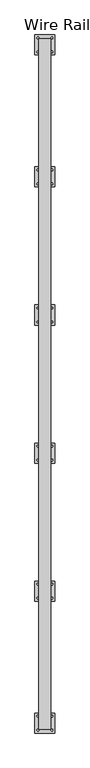
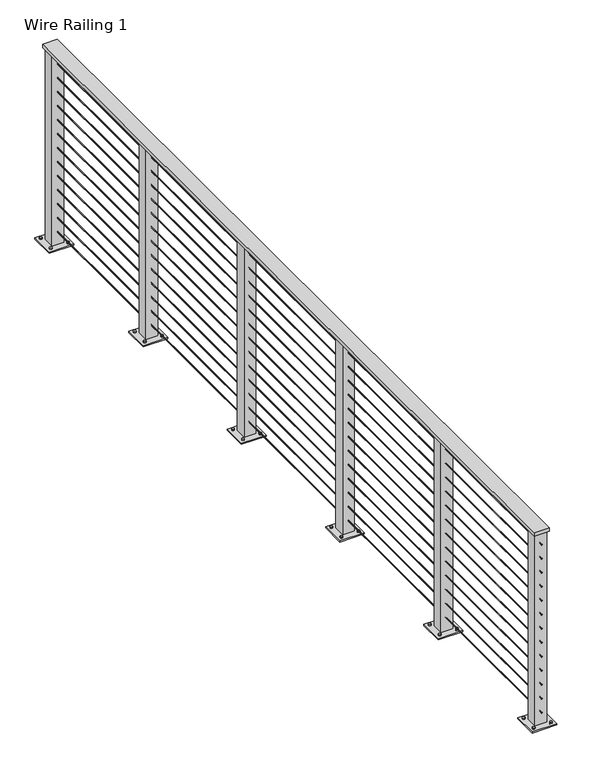
"""IFC4 building model written with IfcOpenShell, lengths in millimetres: railing geometry, Wire Railing 1."""

from ifc_helpers import new_model, si_unit, point, frame, frame_2d, origin, place, context, project, spatial, polyline, circle_curve, trimmed, segment, composite_curve, outline, extrude, source, transform, mapped, element, save


def wire_railing_1_9a376ef2(model_context):
    return source(origin(), model_context, "Body", "SweptSolid", [
        extrude(outline(polyline([(33186.6840778, 35259.9668167), (33262.8840778, 35259.9668167), (33262.8840778, 30878.4668167), (33186.6840778, 30878.4668167), (33186.6840778, 35259.9668167)])), frame((0.0, 0.0, 270300.45), z_axis=(0.0, 0.0, 1.0), x_axis=(1.0, 0.0, 0.0)), (0.0, 0.0, 1.0), 19.05),
        extrude(outline(composite_curve([segment(trimmed(circle_curve(frame_2d((270240.91875, 33224.7840778)), 2.38125), [point((270240.91875, 33227.1653278))], [point((270240.91875, 33222.4028278))], False, "CARTESIAN"), True, "CONTINUOUS"), segment(trimmed(circle_curve(frame_2d((270240.91875, 33224.7840778)), 2.38125), [point((270240.91875, 33222.4028278))], [point((270240.91875, 33227.1653278))], False, "CARTESIAN"), True, "CONTINUOUS")], self_intersect=False)), frame((0.0, 30878.4668167, 0.0), z_axis=(0.0, 1.0, 0.0), x_axis=(0.0, 0.0, 1.0)), (0.0, 0.0, 1.0), 4381.5),
        extrude(outline(composite_curve([segment(trimmed(circle_curve(frame_2d((270164.71875, 33224.7840778)), 2.38125), [point((270164.71875, 33227.1653278))], [point((270164.71875, 33222.4028278))], False, "CARTESIAN"), True, "CONTINUOUS"), segment(trimmed(circle_curve(frame_2d((270164.71875, 33224.7840778)), 2.38125), [point((270164.71875, 33222.4028278))], [point((270164.71875, 33227.1653278))], False, "CARTESIAN"), True, "CONTINUOUS")], self_intersect=False)), frame((0.0, 30878.4668167, 0.0), z_axis=(0.0, 1.0, 0.0), x_axis=(0.0, 0.0, 1.0)), (0.0, 0.0, 1.0), 4381.5),
        extrude(outline(composite_curve([segment(trimmed(circle_curve(frame_2d((270088.51875, 33224.7840778)), 2.38125), [point((270088.51875, 33227.1653278))], [point((270088.51875, 33222.4028278))], False, "CARTESIAN"), True, "CONTINUOUS"), segment(trimmed(circle_curve(frame_2d((270088.51875, 33224.7840778)), 2.38125), [point((270088.51875, 33222.4028278))], [point((270088.51875, 33227.1653278))], False, "CARTESIAN"), True, "CONTINUOUS")], self_intersect=False)), frame((0.0, 30878.4668167, 0.0), z_axis=(0.0, 1.0, 0.0), x_axis=(0.0, 0.0, 1.0)), (0.0, 0.0, 1.0), 4381.5),
        extrude(outline(composite_curve([segment(trimmed(circle_curve(frame_2d((270012.31875, 33224.7840778)), 2.38125), [point((270012.31875, 33227.1653278))], [point((270012.31875, 33222.4028278))], False, "CARTESIAN"), True, "CONTINUOUS"), segment(trimmed(circle_curve(frame_2d((270012.31875, 33224.7840778)), 2.38125), [point((270012.31875, 33222.4028278))], [point((270012.31875, 33227.1653278))], False, "CARTESIAN"), True, "CONTINUOUS")], self_intersect=False)), frame((0.0, 30878.4668167, 0.0), z_axis=(0.0, 1.0, 0.0), x_axis=(0.0, 0.0, 1.0)), (0.0, 0.0, 1.0), 4381.5),
        extrude(outline(composite_curve([segment(trimmed(circle_curve(frame_2d((269936.11875, 33224.7840778)), 2.38125), [point((269936.11875, 33227.1653278))], [point((269936.11875, 33222.4028278))], False, "CARTESIAN"), True, "CONTINUOUS"), segment(trimmed(circle_curve(frame_2d((269936.11875, 33224.7840778)), 2.38125), [point((269936.11875, 33222.4028278))], [point((269936.11875, 33227.1653278))], False, "CARTESIAN"), True, "CONTINUOUS")], self_intersect=False)), frame((0.0, 30878.4668167, 0.0), z_axis=(0.0, 1.0, 0.0), x_axis=(0.0, 0.0, 1.0)), (0.0, 0.0, 1.0), 4381.5),
        extrude(outline(composite_curve([segment(trimmed(circle_curve(frame_2d((269859.91875, 33224.7840778)), 2.38125), [point((269859.91875, 33227.1653278))], [point((269859.91875, 33222.4028278))], False, "CARTESIAN"), True, "CONTINUOUS"), segment(trimmed(circle_curve(frame_2d((269859.91875, 33224.7840778)), 2.38125), [point((269859.91875, 33222.4028278))], [point((269859.91875, 33227.1653278))], False, "CARTESIAN"), True, "CONTINUOUS")], self_intersect=False)), frame((0.0, 30878.4668167, 0.0), z_axis=(0.0, 1.0, 0.0), x_axis=(0.0, 0.0, 1.0)), (0.0, 0.0, 1.0), 4381.5),
        extrude(outline(composite_curve([segment(trimmed(circle_curve(frame_2d((269783.71875, 33224.7840778)), 2.38125), [point((269783.71875, 33227.1653278))], [point((269783.71875, 33222.4028278))], False, "CARTESIAN"), True, "CONTINUOUS"), segment(trimmed(circle_curve(frame_2d((269783.71875, 33224.7840778)), 2.38125), [point((269783.71875, 33222.4028278))], [point((269783.71875, 33227.1653278))], False, "CARTESIAN"), True, "CONTINUOUS")], self_intersect=False)), frame((0.0, 30878.4668167, 0.0), z_axis=(0.0, 1.0, 0.0), x_axis=(0.0, 0.0, 1.0)), (0.0, 0.0, 1.0), 4381.5),
        extrude(outline(composite_curve([segment(trimmed(circle_curve(frame_2d((269707.51875, 33224.7840778)), 2.38125), [point((269707.51875, 33227.1653278))], [point((269707.51875, 33222.4028278))], False, "CARTESIAN"), True, "CONTINUOUS"), segment(trimmed(circle_curve(frame_2d((269707.51875, 33224.7840778)), 2.38125), [point((269707.51875, 33222.4028278))], [point((269707.51875, 33227.1653278))], False, "CARTESIAN"), True, "CONTINUOUS")], self_intersect=False)), frame((0.0, 30878.4668167, 0.0), z_axis=(0.0, 1.0, 0.0), x_axis=(0.0, 0.0, 1.0)), (0.0, 0.0, 1.0), 4381.5),
        extrude(outline(composite_curve([segment(trimmed(circle_curve(frame_2d((269631.31875, 33224.7840778)), 2.38125), [point((269631.31875, 33227.1653278))], [point((269631.31875, 33222.4028278))], False, "CARTESIAN"), True, "CONTINUOUS"), segment(trimmed(circle_curve(frame_2d((269631.31875, 33224.7840778)), 2.38125), [point((269631.31875, 33222.4028278))], [point((269631.31875, 33227.1653278))], False, "CARTESIAN"), True, "CONTINUOUS")], self_intersect=False)), frame((0.0, 30878.4668167, 0.0), z_axis=(0.0, 1.0, 0.0), x_axis=(0.0, 0.0, 1.0)), (0.0, 0.0, 1.0), 4381.5),
        extrude(outline(composite_curve([segment(trimmed(circle_curve(frame_2d((269555.11875, 33224.7840778)), 2.38125), [point((269555.11875, 33227.1653278))], [point((269555.11875, 33222.4028278))], False, "CARTESIAN"), True, "CONTINUOUS"), segment(trimmed(circle_curve(frame_2d((269555.11875, 33224.7840778)), 2.38125), [point((269555.11875, 33222.4028278))], [point((269555.11875, 33227.1653278))], False, "CARTESIAN"), True, "CONTINUOUS")], self_intersect=False)), frame((0.0, 30878.4668167, 0.0), z_axis=(0.0, 1.0, 0.0), x_axis=(0.0, 0.0, 1.0)), (0.0, 0.0, 1.0), 4381.5),
        extrude(outline(composite_curve([segment(trimmed(circle_curve(frame_2d((269478.91875, 33224.7840778)), 2.38125), [point((269478.91875, 33227.1653278))], [point((269478.91875, 33222.4028278))], False, "CARTESIAN"), True, "CONTINUOUS"), segment(trimmed(circle_curve(frame_2d((269478.91875, 33224.7840778)), 2.38125), [point((269478.91875, 33222.4028278))], [point((269478.91875, 33227.1653278))], False, "CARTESIAN"), True, "CONTINUOUS")], self_intersect=False)), frame((0.0, 30878.4668167, 0.0), z_axis=(0.0, 1.0, 0.0), x_axis=(0.0, 0.0, 1.0)), (0.0, 0.0, 1.0), 4381.5),
        extrude(outline(composite_curve([segment(trimmed(circle_curve(frame_2d((269402.71875, 33224.7840778)), 2.38125), [point((269402.71875, 33227.1653278))], [point((269402.71875, 33222.4028278))], False, "CARTESIAN"), True, "CONTINUOUS"), segment(trimmed(circle_curve(frame_2d((269402.71875, 33224.7840778)), 2.38125), [point((269402.71875, 33222.4028278))], [point((269402.71875, 33227.1653278))], False, "CARTESIAN"), True, "CONTINUOUS")], self_intersect=False)), frame((0.0, 30878.4668167, 0.0), z_axis=(0.0, 1.0, 0.0), x_axis=(0.0, 0.0, 1.0)), (0.0, 0.0, 1.0), 4381.5),
        extrude(outline(composite_curve([segment(trimmed(circle_curve(frame_2d((269326.51875, 33224.7840778)), 2.38125), [point((269326.51875, 33227.1653278))], [point((269326.51875, 33222.4028278))], False, "CARTESIAN"), True, "CONTINUOUS"), segment(trimmed(circle_curve(frame_2d((269326.51875, 33224.7840778)), 2.38125), [point((269326.51875, 33222.4028278))], [point((269326.51875, 33227.1653278))], False, "CARTESIAN"), True, "CONTINUOUS")], self_intersect=False)), frame((0.0, 30878.4668167, 0.0), z_axis=(0.0, 1.0, 0.0), x_axis=(0.0, 0.0, 1.0)), (0.0, 0.0, 1.0), 4381.5),
        extrude(outline(composite_curve([segment(trimmed(circle_curve(frame_2d((33180.3340778, 31799.2168167)), 6.35), [point((33173.9840778, 31799.2168167))], [point((33186.6840778, 31799.2168167))], False, "CARTESIAN"), True, "CONTINUOUS"), segment(trimmed(circle_curve(frame_2d((33180.3340778, 31799.2168167)), 6.35), [point((33186.6840778, 31799.2168167))], [point((33173.9840778, 31799.2168167))], False, "CARTESIAN"), True, "CONTINUOUS")], self_intersect=False)), frame((0.0, 0.0, 269252.7), z_axis=(0.0, 0.0, 1.0), x_axis=(1.0, 0.0, 0.0)), (0.0, 0.0, 1.0), 12.7),
        extrude(outline(composite_curve([segment(trimmed(circle_curve(frame_2d((33269.2340778, 31799.2168167)), 6.35), [point((33262.8840778, 31799.2168167))], [point((33275.5840778, 31799.2168167))], False, "CARTESIAN"), True, "CONTINUOUS"), segment(trimmed(circle_curve(frame_2d((33269.2340778, 31799.2168167)), 6.35), [point((33275.5840778, 31799.2168167))], [point((33262.8840778, 31799.2168167))], False, "CARTESIAN"), True, "CONTINUOUS")], self_intersect=False)), frame((0.0, 0.0, 269252.7), z_axis=(0.0, 0.0, 1.0), x_axis=(1.0, 0.0, 0.0)), (0.0, 0.0, 1.0), 12.7),
        extrude(outline(composite_curve([segment(trimmed(circle_curve(frame_2d((33180.3340778, 31710.3168167)), 6.35), [point((33173.9840778, 31710.3168167))], [point((33186.6840778, 31710.3168167))], False, "CARTESIAN"), True, "CONTINUOUS"), segment(trimmed(circle_curve(frame_2d((33180.3340778, 31710.3168167)), 6.35), [point((33186.6840778, 31710.3168167))], [point((33173.9840778, 31710.3168167))], False, "CARTESIAN"), True, "CONTINUOUS")], self_intersect=False)), frame((0.0, 0.0, 269252.7), z_axis=(0.0, 0.0, 1.0), x_axis=(1.0, 0.0, 0.0)), (0.0, 0.0, 1.0), 12.7),
        extrude(outline(composite_curve([segment(trimmed(circle_curve(frame_2d((33269.2340778, 31710.3168167)), 6.35), [point((33262.8840778, 31710.3168167))], [point((33275.5840778, 31710.3168167))], False, "CARTESIAN"), True, "CONTINUOUS"), segment(trimmed(circle_curve(frame_2d((33269.2340778, 31710.3168167)), 6.35), [point((33275.5840778, 31710.3168167))], [point((33262.8840778, 31710.3168167))], False, "CARTESIAN"), True, "CONTINUOUS")], self_intersect=False)), frame((0.0, 0.0, 269252.7), z_axis=(0.0, 0.0, 1.0), x_axis=(1.0, 0.0, 0.0)), (0.0, 0.0, 1.0), 12.7),
        extrude(outline(polyline([(33288.2840778, 31818.2668167), (33288.2840778, 31691.2668167), (33161.2840778, 31691.2668167), (33161.2840778, 31818.2668167), (33288.2840778, 31818.2668167)])), frame((0.0, 0.0, 269252.7), z_axis=(0.0, 0.0, 1.0), x_axis=(1.0, 0.0, 0.0)), (0.0, 0.0, 1.0), 6.35),
        extrude(outline(polyline([(33254.9465778, 31784.9293167), (33254.9465778, 31724.6043167), (33194.6215778, 31724.6043167), (33194.6215778, 31784.9293167), (33254.9465778, 31784.9293167)]), holes=[polyline([(33248.5965778, 31778.5793167), (33200.9715778, 31778.5793167), (33200.9715778, 31730.9543167), (33248.5965778, 31730.9543167), (33248.5965778, 31778.5793167)])]), frame((0.0, 0.0, 269252.7), z_axis=(0.0, 0.0, 1.0), x_axis=(1.0, 0.0, 0.0)), (0.0, 0.0, 1.0), 1047.75),
        extrude(outline(composite_curve([segment(trimmed(circle_curve(frame_2d((33180.3340778, 32675.5168167)), 6.35), [point((33173.9840778, 32675.5168167))], [point((33186.6840778, 32675.5168167))], False, "CARTESIAN"), True, "CONTINUOUS"), segment(trimmed(circle_curve(frame_2d((33180.3340778, 32675.5168167)), 6.35), [point((33186.6840778, 32675.5168167))], [point((33173.9840778, 32675.5168167))], False, "CARTESIAN"), True, "CONTINUOUS")], self_intersect=False)), frame((0.0, 0.0, 269252.7), z_axis=(0.0, 0.0, 1.0), x_axis=(1.0, 0.0, 0.0)), (0.0, 0.0, 1.0), 12.7),
        extrude(outline(composite_curve([segment(trimmed(circle_curve(frame_2d((33269.2340778, 32675.5168167)), 6.35), [point((33262.8840778, 32675.5168167))], [point((33275.5840778, 32675.5168167))], False, "CARTESIAN"), True, "CONTINUOUS"), segment(trimmed(circle_curve(frame_2d((33269.2340778, 32675.5168167)), 6.35), [point((33275.5840778, 32675.5168167))], [point((33262.8840778, 32675.5168167))], False, "CARTESIAN"), True, "CONTINUOUS")], self_intersect=False)), frame((0.0, 0.0, 269252.7), z_axis=(0.0, 0.0, 1.0), x_axis=(1.0, 0.0, 0.0)), (0.0, 0.0, 1.0), 12.7),
        extrude(outline(composite_curve([segment(trimmed(circle_curve(frame_2d((33180.3340778, 32586.6168167)), 6.35), [point((33173.9840778, 32586.6168167))], [point((33186.6840778, 32586.6168167))], False, "CARTESIAN"), True, "CONTINUOUS"), segment(trimmed(circle_curve(frame_2d((33180.3340778, 32586.6168167)), 6.35), [point((33186.6840778, 32586.6168167))], [point((33173.9840778, 32586.6168167))], False, "CARTESIAN"), True, "CONTINUOUS")], self_intersect=False)), frame((0.0, 0.0, 269252.7), z_axis=(0.0, 0.0, 1.0), x_axis=(1.0, 0.0, 0.0)), (0.0, 0.0, 1.0), 12.7),
        extrude(outline(composite_curve([segment(trimmed(circle_curve(frame_2d((33269.2340778, 32586.6168167)), 6.35), [point((33262.8840778, 32586.6168167))], [point((33275.5840778, 32586.6168167))], False, "CARTESIAN"), True, "CONTINUOUS"), segment(trimmed(circle_curve(frame_2d((33269.2340778, 32586.6168167)), 6.35), [point((33275.5840778, 32586.6168167))], [point((33262.8840778, 32586.6168167))], False, "CARTESIAN"), True, "CONTINUOUS")], self_intersect=False)), frame((0.0, 0.0, 269252.7), z_axis=(0.0, 0.0, 1.0), x_axis=(1.0, 0.0, 0.0)), (0.0, 0.0, 1.0), 12.7),
        extrude(outline(polyline([(33288.2840778, 32694.5668167), (33288.2840778, 32567.5668167), (33161.2840778, 32567.5668167), (33161.2840778, 32694.5668167), (33288.2840778, 32694.5668167)])), frame((0.0, 0.0, 269252.7), z_axis=(0.0, 0.0, 1.0), x_axis=(1.0, 0.0, 0.0)), (0.0, 0.0, 1.0), 6.35),
        extrude(outline(polyline([(33254.9465778, 32661.2293167), (33254.9465778, 32600.9043167), (33194.6215778, 32600.9043167), (33194.6215778, 32661.2293167), (33254.9465778, 32661.2293167)]), holes=[polyline([(33248.5965778, 32654.8793167), (33200.9715778, 32654.8793167), (33200.9715778, 32607.2543167), (33248.5965778, 32607.2543167), (33248.5965778, 32654.8793167)])]), frame((0.0, 0.0, 269252.7), z_axis=(0.0, 0.0, 1.0), x_axis=(1.0, 0.0, 0.0)), (0.0, 0.0, 1.0), 1047.75),
        extrude(outline(composite_curve([segment(trimmed(circle_curve(frame_2d((33180.3340778, 33551.8168167)), 6.35), [point((33173.9840778, 33551.8168167))], [point((33186.6840778, 33551.8168167))], False, "CARTESIAN"), True, "CONTINUOUS"), segment(trimmed(circle_curve(frame_2d((33180.3340778, 33551.8168167)), 6.35), [point((33186.6840778, 33551.8168167))], [point((33173.9840778, 33551.8168167))], False, "CARTESIAN"), True, "CONTINUOUS")], self_intersect=False)), frame((0.0, 0.0, 269252.7), z_axis=(0.0, 0.0, 1.0), x_axis=(1.0, 0.0, 0.0)), (0.0, 0.0, 1.0), 12.7),
        extrude(outline(composite_curve([segment(trimmed(circle_curve(frame_2d((33269.2340778, 33551.8168167)), 6.35), [point((33262.8840778, 33551.8168167))], [point((33275.5840778, 33551.8168167))], False, "CARTESIAN"), True, "CONTINUOUS"), segment(trimmed(circle_curve(frame_2d((33269.2340778, 33551.8168167)), 6.35), [point((33275.5840778, 33551.8168167))], [point((33262.8840778, 33551.8168167))], False, "CARTESIAN"), True, "CONTINUOUS")], self_intersect=False)), frame((0.0, 0.0, 269252.7), z_axis=(0.0, 0.0, 1.0), x_axis=(1.0, 0.0, 0.0)), (0.0, 0.0, 1.0), 12.7),
        extrude(outline(composite_curve([segment(trimmed(circle_curve(frame_2d((33180.3340778, 33462.9168167)), 6.35), [point((33173.9840778, 33462.9168167))], [point((33186.6840778, 33462.9168167))], False, "CARTESIAN"), True, "CONTINUOUS"), segment(trimmed(circle_curve(frame_2d((33180.3340778, 33462.9168167)), 6.35), [point((33186.6840778, 33462.9168167))], [point((33173.9840778, 33462.9168167))], False, "CARTESIAN"), True, "CONTINUOUS")], self_intersect=False)), frame((0.0, 0.0, 269252.7), z_axis=(0.0, 0.0, 1.0), x_axis=(1.0, 0.0, 0.0)), (0.0, 0.0, 1.0), 12.7),
        extrude(outline(composite_curve([segment(trimmed(circle_curve(frame_2d((33269.2340778, 33462.9168167)), 6.35), [point((33262.8840778, 33462.9168167))], [point((33275.5840778, 33462.9168167))], False, "CARTESIAN"), True, "CONTINUOUS"), segment(trimmed(circle_curve(frame_2d((33269.2340778, 33462.9168167)), 6.35), [point((33275.5840778, 33462.9168167))], [point((33262.8840778, 33462.9168167))], False, "CARTESIAN"), True, "CONTINUOUS")], self_intersect=False)), frame((0.0, 0.0, 269252.7), z_axis=(0.0, 0.0, 1.0), x_axis=(1.0, 0.0, 0.0)), (0.0, 0.0, 1.0), 12.7),
        extrude(outline(polyline([(33288.2840778, 33570.8668167), (33288.2840778, 33443.8668167), (33161.2840778, 33443.8668167), (33161.2840778, 33570.8668167), (33288.2840778, 33570.8668167)])), frame((0.0, 0.0, 269252.7), z_axis=(0.0, 0.0, 1.0), x_axis=(1.0, 0.0, 0.0)), (0.0, 0.0, 1.0), 6.35),
        extrude(outline(polyline([(33254.9465778, 33537.5293167), (33254.9465778, 33477.2043167), (33194.6215778, 33477.2043167), (33194.6215778, 33537.5293167), (33254.9465778, 33537.5293167)]), holes=[polyline([(33248.5965778, 33531.1793167), (33200.9715778, 33531.1793167), (33200.9715778, 33483.5543167), (33248.5965778, 33483.5543167), (33248.5965778, 33531.1793167)])]), frame((0.0, 0.0, 269252.7), z_axis=(0.0, 0.0, 1.0), x_axis=(1.0, 0.0, 0.0)), (0.0, 0.0, 1.0), 1047.75),
        extrude(outline(composite_curve([segment(trimmed(circle_curve(frame_2d((33180.3340778, 34428.1168167)), 6.35), [point((33173.9840778, 34428.1168167))], [point((33186.6840778, 34428.1168167))], False, "CARTESIAN"), True, "CONTINUOUS"), segment(trimmed(circle_curve(frame_2d((33180.3340778, 34428.1168167)), 6.35), [point((33186.6840778, 34428.1168167))], [point((33173.9840778, 34428.1168167))], False, "CARTESIAN"), True, "CONTINUOUS")], self_intersect=False)), frame((0.0, 0.0, 269252.7), z_axis=(0.0, 0.0, 1.0), x_axis=(1.0, 0.0, 0.0)), (0.0, 0.0, 1.0), 12.7),
        extrude(outline(composite_curve([segment(trimmed(circle_curve(frame_2d((33269.2340778, 34428.1168167)), 6.35), [point((33262.8840778, 34428.1168167))], [point((33275.5840778, 34428.1168167))], False, "CARTESIAN"), True, "CONTINUOUS"), segment(trimmed(circle_curve(frame_2d((33269.2340778, 34428.1168167)), 6.35), [point((33275.5840778, 34428.1168167))], [point((33262.8840778, 34428.1168167))], False, "CARTESIAN"), True, "CONTINUOUS")], self_intersect=False)), frame((0.0, 0.0, 269252.7), z_axis=(0.0, 0.0, 1.0), x_axis=(1.0, 0.0, 0.0)), (0.0, 0.0, 1.0), 12.7),
        extrude(outline(composite_curve([segment(trimmed(circle_curve(frame_2d((33180.3340778, 34339.2168167)), 6.35), [point((33173.9840778, 34339.2168167))], [point((33186.6840778, 34339.2168167))], False, "CARTESIAN"), True, "CONTINUOUS"), segment(trimmed(circle_curve(frame_2d((33180.3340778, 34339.2168167)), 6.35), [point((33186.6840778, 34339.2168167))], [point((33173.9840778, 34339.2168167))], False, "CARTESIAN"), True, "CONTINUOUS")], self_intersect=False)), frame((0.0, 0.0, 269252.7), z_axis=(0.0, 0.0, 1.0), x_axis=(1.0, 0.0, 0.0)), (0.0, 0.0, 1.0), 12.7),
        extrude(outline(composite_curve([segment(trimmed(circle_curve(frame_2d((33269.2340778, 34339.2168167)), 6.35), [point((33262.8840778, 34339.2168167))], [point((33275.5840778, 34339.2168167))], False, "CARTESIAN"), True, "CONTINUOUS"), segment(trimmed(circle_curve(frame_2d((33269.2340778, 34339.2168167)), 6.35), [point((33275.5840778, 34339.2168167))], [point((33262.8840778, 34339.2168167))], False, "CARTESIAN"), True, "CONTINUOUS")], self_intersect=False)), frame((0.0, 0.0, 269252.7), z_axis=(0.0, 0.0, 1.0), x_axis=(1.0, 0.0, 0.0)), (0.0, 0.0, 1.0), 12.7),
        extrude(outline(polyline([(33288.2840778, 34447.1668167), (33288.2840778, 34320.1668167), (33161.2840778, 34320.1668167), (33161.2840778, 34447.1668167), (33288.2840778, 34447.1668167)])), frame((0.0, 0.0, 269252.7), z_axis=(0.0, 0.0, 1.0), x_axis=(1.0, 0.0, 0.0)), (0.0, 0.0, 1.0), 6.35),
        extrude(outline(polyline([(33254.9465778, 34413.8293167), (33254.9465778, 34353.5043167), (33194.6215778, 34353.5043167), (33194.6215778, 34413.8293167), (33254.9465778, 34413.8293167)]), holes=[polyline([(33248.5965778, 34407.4793167), (33200.9715778, 34407.4793167), (33200.9715778, 34359.8543167), (33248.5965778, 34359.8543167), (33248.5965778, 34407.4793167)])]), frame((0.0, 0.0, 269252.7), z_axis=(0.0, 0.0, 1.0), x_axis=(1.0, 0.0, 0.0)), (0.0, 0.0, 1.0), 1047.75),
        extrude(outline(composite_curve([segment(trimmed(circle_curve(frame_2d((33180.3340778, 30961.0168167)), 6.35), [point((33173.9840778, 30961.0168167))], [point((33186.6840778, 30961.0168167))], False, "CARTESIAN"), True, "CONTINUOUS"), segment(trimmed(circle_curve(frame_2d((33180.3340778, 30961.0168167)), 6.35), [point((33186.6840778, 30961.0168167))], [point((33173.9840778, 30961.0168167))], False, "CARTESIAN"), True, "CONTINUOUS")], self_intersect=False)), frame((0.0, 0.0, 269252.7), z_axis=(0.0, 0.0, 1.0), x_axis=(1.0, 0.0, 0.0)), (0.0, 0.0, 1.0), 12.7),
        extrude(outline(composite_curve([segment(trimmed(circle_curve(frame_2d((33269.2340778, 30961.0168167)), 6.35), [point((33262.8840778, 30961.0168167))], [point((33275.5840778, 30961.0168167))], False, "CARTESIAN"), True, "CONTINUOUS"), segment(trimmed(circle_curve(frame_2d((33269.2340778, 30961.0168167)), 6.35), [point((33275.5840778, 30961.0168167))], [point((33262.8840778, 30961.0168167))], False, "CARTESIAN"), True, "CONTINUOUS")], self_intersect=False)), frame((0.0, 0.0, 269252.7), z_axis=(0.0, 0.0, 1.0), x_axis=(1.0, 0.0, 0.0)), (0.0, 0.0, 1.0), 12.7),
        extrude(outline(composite_curve([segment(trimmed(circle_curve(frame_2d((33180.3340778, 30872.1168167)), 6.35), [point((33173.9840778, 30872.1168167))], [point((33186.6840778, 30872.1168167))], False, "CARTESIAN"), True, "CONTINUOUS"), segment(trimmed(circle_curve(frame_2d((33180.3340778, 30872.1168167)), 6.35), [point((33186.6840778, 30872.1168167))], [point((33173.9840778, 30872.1168167))], False, "CARTESIAN"), True, "CONTINUOUS")], self_intersect=False)), frame((0.0, 0.0, 269252.7), z_axis=(0.0, 0.0, 1.0), x_axis=(1.0, 0.0, 0.0)), (0.0, 0.0, 1.0), 12.7),
        extrude(outline(composite_curve([segment(trimmed(circle_curve(frame_2d((33269.2340778, 30872.1168167)), 6.35), [point((33262.8840778, 30872.1168167))], [point((33275.5840778, 30872.1168167))], False, "CARTESIAN"), True, "CONTINUOUS"), segment(trimmed(circle_curve(frame_2d((33269.2340778, 30872.1168167)), 6.35), [point((33275.5840778, 30872.1168167))], [point((33262.8840778, 30872.1168167))], False, "CARTESIAN"), True, "CONTINUOUS")], self_intersect=False)), frame((0.0, 0.0, 269252.7), z_axis=(0.0, 0.0, 1.0), x_axis=(1.0, 0.0, 0.0)), (0.0, 0.0, 1.0), 12.7),
        extrude(outline(polyline([(33288.2840778, 30980.0668167), (33288.2840778, 30853.0668167), (33161.2840778, 30853.0668167), (33161.2840778, 30980.0668167), (33288.2840778, 30980.0668167)])), frame((0.0, 0.0, 269252.7), z_axis=(0.0, 0.0, 1.0), x_axis=(1.0, 0.0, 0.0)), (0.0, 0.0, 1.0), 6.35),
        extrude(outline(polyline([(33254.9465778, 30946.7293167), (33254.9465778, 30886.4043167), (33194.6215778, 30886.4043167), (33194.6215778, 30946.7293167), (33254.9465778, 30946.7293167)]), holes=[polyline([(33248.5965778, 30940.3793167), (33200.9715778, 30940.3793167), (33200.9715778, 30892.7543167), (33248.5965778, 30892.7543167), (33248.5965778, 30940.3793167)])]), frame((0.0, 0.0, 269252.7), z_axis=(0.0, 0.0, 1.0), x_axis=(1.0, 0.0, 0.0)), (0.0, 0.0, 1.0), 1047.75),
        extrude(outline(composite_curve([segment(trimmed(circle_curve(frame_2d((33180.3340778, 35266.3168167)), 6.35), [point((33173.9840778, 35266.3168167))], [point((33186.6840778, 35266.3168167))], False, "CARTESIAN"), True, "CONTINUOUS"), segment(trimmed(circle_curve(frame_2d((33180.3340778, 35266.3168167)), 6.35), [point((33186.6840778, 35266.3168167))], [point((33173.9840778, 35266.3168167))], False, "CARTESIAN"), True, "CONTINUOUS")], self_intersect=False)), frame((0.0, 0.0, 269252.7), z_axis=(0.0, 0.0, 1.0), x_axis=(1.0, 0.0, 0.0)), (0.0, 0.0, 1.0), 12.7),
        extrude(outline(composite_curve([segment(trimmed(circle_curve(frame_2d((33269.2340778, 35266.3168167)), 6.35), [point((33262.8840778, 35266.3168167))], [point((33275.5840778, 35266.3168167))], False, "CARTESIAN"), True, "CONTINUOUS"), segment(trimmed(circle_curve(frame_2d((33269.2340778, 35266.3168167)), 6.35), [point((33275.5840778, 35266.3168167))], [point((33262.8840778, 35266.3168167))], False, "CARTESIAN"), True, "CONTINUOUS")], self_intersect=False)), frame((0.0, 0.0, 269252.7), z_axis=(0.0, 0.0, 1.0), x_axis=(1.0, 0.0, 0.0)), (0.0, 0.0, 1.0), 12.7),
        extrude(outline(composite_curve([segment(trimmed(circle_curve(frame_2d((33180.3340778, 35177.4168167)), 6.35), [point((33173.9840778, 35177.4168167))], [point((33186.6840778, 35177.4168167))], False, "CARTESIAN"), True, "CONTINUOUS"), segment(trimmed(circle_curve(frame_2d((33180.3340778, 35177.4168167)), 6.35), [point((33186.6840778, 35177.4168167))], [point((33173.9840778, 35177.4168167))], False, "CARTESIAN"), True, "CONTINUOUS")], self_intersect=False)), frame((0.0, 0.0, 269252.7), z_axis=(0.0, 0.0, 1.0), x_axis=(1.0, 0.0, 0.0)), (0.0, 0.0, 1.0), 12.7),
        extrude(outline(composite_curve([segment(trimmed(circle_curve(frame_2d((33269.2340778, 35177.4168167)), 6.35), [point((33262.8840778, 35177.4168167))], [point((33275.5840778, 35177.4168167))], False, "CARTESIAN"), True, "CONTINUOUS"), segment(trimmed(circle_curve(frame_2d((33269.2340778, 35177.4168167)), 6.35), [point((33275.5840778, 35177.4168167))], [point((33262.8840778, 35177.4168167))], False, "CARTESIAN"), True, "CONTINUOUS")], self_intersect=False)), frame((0.0, 0.0, 269252.7), z_axis=(0.0, 0.0, 1.0), x_axis=(1.0, 0.0, 0.0)), (0.0, 0.0, 1.0), 12.7),
        extrude(outline(polyline([(33288.2840778, 35285.3668167), (33288.2840778, 35158.3668167), (33161.2840778, 35158.3668167), (33161.2840778, 35285.3668167), (33288.2840778, 35285.3668167)])), frame((0.0, 0.0, 269252.7), z_axis=(0.0, 0.0, 1.0), x_axis=(1.0, 0.0, 0.0)), (0.0, 0.0, 1.0), 6.35),
        extrude(outline(polyline([(33254.9465778, 35252.0293167), (33254.9465778, 35191.7043167), (33194.6215778, 35191.7043167), (33194.6215778, 35252.0293167), (33254.9465778, 35252.0293167)]), holes=[polyline([(33248.5965778, 35245.6793167), (33200.9715778, 35245.6793167), (33200.9715778, 35198.0543167), (33248.5965778, 35198.0543167), (33248.5965778, 35245.6793167)])]), frame((0.0, 0.0, 269252.7), z_axis=(0.0, 0.0, 1.0), x_axis=(1.0, 0.0, 0.0)), (0.0, 0.0, 1.0), 1047.75),
    ])


if __name__ == "__main__":
    model = new_model("IFC4")
    model_context = context("Model", 3, world=origin())
    ifc_project = project(units=[si_unit("LENGTHUNIT", "METRE", prefix="MILLI")], contexts=[model_context])
    site = spatial("IfcSite", under=ifc_project)
    building = spatial("IfcBuilding", under=site)
    placement = place(None, origin())
    wire_railing_1_shape = wire_railing_1_9a376ef2(model_context)
    element("IfcRailing", 1, ObjectType="Wire Railing 1", at=placement, inside=building, context=model_context, shape_type="MappedRepresentation", body=[
        mapped(wire_railing_1_shape, transform((0.0, 0.0, 0.0), x_axis=(1.0, 0.0, 0.0), y_axis=(0.0, 1.0, 0.0), z_axis=(0.0, 0.0, 1.0))),
    ])
    save(model, "model.ifc")

# Revit data of these elements
# Element 1 (IfcRailing, "Wire Railing 1")
#   Materials on its faces: "WIRE RAILING"
# Materials
#   "WIRE RAILING": class "Metal", colour RGB 244 244 244, transparency 0, Manufacturer = "Kawneer", URL = "http://www.kawneer.com/kawneer/north_america/en/home.asp", Cost = 0
